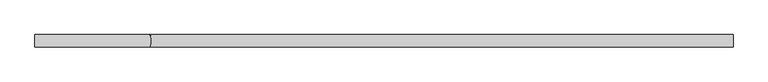
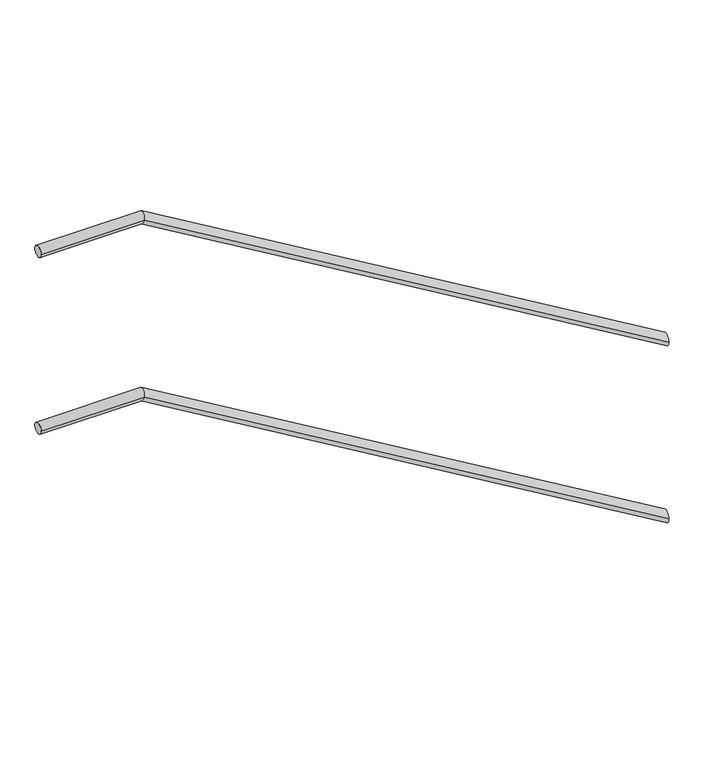
"""IFC4 building model written with IfcOpenShell, lengths in millimetres: railing geometry."""

from ifc_helpers import new_model, si_unit, frame, origin, place, context, project, spatial, circle_curve, ellipse_curve, source, transform, mapped, element, save
from ifc_brep_helpers import plane_surface, cylinder_surface, advanced_brep


def railing_cd17721a(model_context):
    return source(origin(), model_context, "Body", "AdvancedBrep", [
        advanced_brep(
        [(29704.7, -1668.0791411, 899.2104532), (29704.7, -1698.0791411, 899.2104532), (28300.5735614, -1698.0791411, 1735.0), (28300.5735614, -1668.0791411, 1735.0), (28024.7, -1668.0791411, 1735.0), (28024.7, -1698.0791411, 1735.0)],
        [
            (0, 1, ellipse_curve(frame((29704.7, -1683.0791411, 899.2104532), z_axis=(1.0, 0.0, 0.0), x_axis=(0.0, 0.0, -1.0)), 17.4562134, 15.0)),
            (1, 0, ellipse_curve(frame((29704.7, -1683.0791411, 899.2104532), z_axis=(1.0, 0.0, 0.0), x_axis=(0.0, 0.0, -1.0)), 17.4562134, 15.0)),
            (1, 2),
            (2, 3, ellipse_curve(frame((28300.5735614, -1683.0791411, 1735.0), z_axis=(0.9641817474962145, 0.0, -0.2652424509673106), x_axis=(-0.26524245096731125, 0.0, -0.9641817474962143)), 15.5572329, 15.0)),
            (3, 0),
            (3, 2, ellipse_curve(frame((28300.5735614, -1683.0791411, 1735.0), z_axis=(0.9641817474962145, 0.0, -0.2652424509673106), x_axis=(-0.26524245096731125, 0.0, -0.9641817474962143)), 15.5572329, 15.0)),
            (4, 5, circle_curve(frame((28024.7, -1683.0791411, 1735.0), z_axis=(-1.0, 0.0, 0.0), x_axis=(0.0, -1.0, 0.0)), 15.0)),
            (5, 4, circle_curve(frame((28024.7, -1683.0791411, 1735.0), z_axis=(-1.0, 0.0, 0.0), x_axis=(0.0, -1.0, 0.0)), 15.0)),
            (2, 5),
            (4, 3),
        ],
        [
            plane_surface(frame((29704.7, -1683.0791411, 916.6666667), z_axis=(1.0, 0.0, 0.0), x_axis=(0.0, -1.0, 0.0))),
            cylinder_surface(frame((29697.0277421, -1683.0791411, 903.7772734), z_axis=(0.8592928844097079, 0.0, -0.5114838597676808), x_axis=(0.0, -1.0, 0.0)), 15.0),
            plane_surface(frame((28024.7, -1683.0791411, 1750.0), z_axis=(-1.0, 0.0, 0.0), x_axis=(0.0, -1.0, 0.0))),
            cylinder_surface(frame((28304.7, -1683.0791411, 1735.0), z_axis=(1.0, 0.0, 0.0), x_axis=(0.0, -1.0, 0.0)), 15.0),
        ],
        [
            (0, [[1, 2]]),
            (1, [[-2, 3, 4, 5]]),
            (1, [[-1, -5, 6, -3]]),
            (2, [[7, 8]]),
            (3, [[-4, 9, -7, 10]]),
            (3, [[-6, -10, -8, -9]]),
        ],
    ),
        advanced_brep(
        [(29704.7, -1668.0791411, 1399.2104532), (29704.7, -1698.0791411, 1399.2104532), (28300.5735614, -1698.0791411, 2235.0), (28300.5735614, -1668.0791411, 2235.0), (28024.7, -1668.0791411, 2235.0), (28024.7, -1698.0791411, 2235.0)],
        [
            (0, 1, ellipse_curve(frame((29704.7, -1683.0791411, 1399.2104532), z_axis=(1.0, 0.0, 0.0), x_axis=(0.0, 0.0, -1.0)), 17.4562134, 15.0)),
            (1, 0, ellipse_curve(frame((29704.7, -1683.0791411, 1399.2104532), z_axis=(1.0, 0.0, 0.0), x_axis=(0.0, 0.0, -1.0)), 17.4562134, 15.0)),
            (1, 2),
            (2, 3, ellipse_curve(frame((28300.5735614, -1683.0791411, 2235.0), z_axis=(0.9641817474962145, 0.0, -0.2652424509673106), x_axis=(-0.26524245096731125, 0.0, -0.9641817474962143)), 15.5572329, 15.0)),
            (3, 0),
            (3, 2, ellipse_curve(frame((28300.5735614, -1683.0791411, 2235.0), z_axis=(0.9641817474962145, 0.0, -0.2652424509673106), x_axis=(-0.26524245096731125, 0.0, -0.9641817474962143)), 15.5572329, 15.0)),
            (4, 5, circle_curve(frame((28024.7, -1683.0791411, 2235.0), z_axis=(-1.0, 0.0, 0.0), x_axis=(0.0, -1.0, 0.0)), 15.0)),
            (5, 4, circle_curve(frame((28024.7, -1683.0791411, 2235.0), z_axis=(-1.0, 0.0, 0.0), x_axis=(0.0, -1.0, 0.0)), 15.0)),
            (2, 5),
            (4, 3),
        ],
        [
            plane_surface(frame((29704.7, -1683.0791411, 1416.6666667), z_axis=(1.0, 0.0, 0.0), x_axis=(0.0, -1.0, 0.0))),
            cylinder_surface(frame((29697.0277421, -1683.0791411, 1403.7772734), z_axis=(0.8592928844097079, 0.0, -0.5114838597676808), x_axis=(0.0, -1.0, 0.0)), 15.0),
            plane_surface(frame((28024.7, -1683.0791411, 2250.0), z_axis=(-1.0, 0.0, 0.0), x_axis=(0.0, -1.0, 0.0))),
            cylinder_surface(frame((28304.7, -1683.0791411, 2235.0), z_axis=(1.0, 0.0, 0.0), x_axis=(0.0, -1.0, 0.0)), 15.0),
        ],
        [
            (0, [[1, 2]]),
            (1, [[-2, 3, 4, 5]]),
            (1, [[-1, -5, 6, -3]]),
            (2, [[7, 8]]),
            (3, [[-4, 9, -7, 10]]),
            (3, [[-6, -10, -8, -9]]),
        ],
    ),
    ])


if __name__ == "__main__":
    model = new_model("IFC4")
    model_context = context("Model", 3, world=origin())
    ifc_project = project(units=[si_unit("LENGTHUNIT", "METRE", prefix="MILLI")], contexts=[model_context])
    site = spatial("IfcSite", under=ifc_project)
    building = spatial("IfcBuilding", under=site)
    placement = place(None, origin())
    railing_shape = railing_cd17721a(model_context)
    element("IfcRailing", 1, at=placement, inside=building, context=model_context, shape_type="MappedRepresentation", body=[
        mapped(railing_shape, transform((0.0, 0.0, 0.0), x_axis=(1.0, 0.0, 0.0), y_axis=(0.0, 1.0, 0.0), z_axis=(0.0, 0.0, 1.0))),
    ])
    save(model, "model.ifc")
